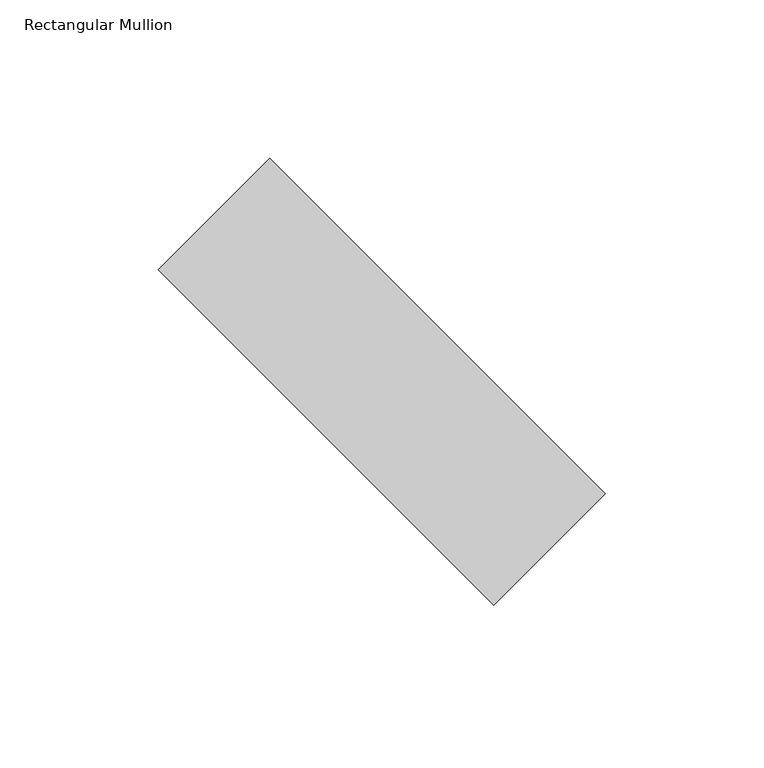
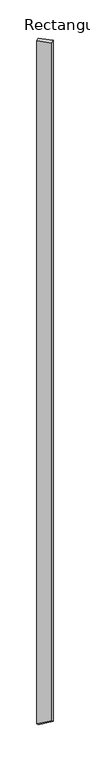
"""IFC4 building model written with IfcOpenShell, lengths in millimetres: member geometry, Rectangular Mullion : tilted mullions."""

from ifc_helpers import new_model, si_unit, origin, place, context, project, spatial, faceted_brep, source, transform, mapped, element, save


def rectangular_mullion_086599bb(model_context):
    return source(origin(), model_context, "Body", "Brep", [
        faceted_brep([(-35.3553391, 70.7106781, 0.0), (-70.7106781, 35.3553391, 0.0), (35.3553391, -70.7106781, 0.0), (70.7106781, -35.3553391, 0.0), (-35.3553391, 70.7106781, -8054.9932319), (-70.7106781, 35.3553391, -8010.0057806), (35.3553391, -70.7106781, -7944.5446238), (70.7106781, -35.3553391, -7989.532075)], [[[0, 1, 2, 3]], [[1, 0, 4, 5]], [[2, 1, 5, 6]], [[3, 2, 6, 7]], [[0, 3, 7, 4]], [[4, 7, 6, 5]]]),
    ])


if __name__ == "__main__":
    model = new_model("IFC4")
    model_context = context("Model", 3, world=origin())
    ifc_project = project(units=[si_unit("LENGTHUNIT", "METRE", prefix="MILLI")], contexts=[model_context])
    site = spatial("IfcSite", under=ifc_project)
    building = spatial("IfcBuilding", under=site)
    placement = place(None, origin())
    rectangular_mullion_shape = rectangular_mullion_086599bb(model_context)
    element("IfcMember", 1, ObjectType="Rectangular Mullion : tilted mullions", at=placement, inside=building, context=model_context, shape_type="MappedRepresentation", body=[
        mapped(rectangular_mullion_shape, transform((0.0, 0.0, 0.0), x_axis=(1.0, 0.0, 0.0), y_axis=(0.0, 1.0, 0.0), z_axis=(0.0, 0.0, 1.0))),
    ])
    save(model, "model.ifc")

# Revit data of these elements
# Type "Rectangular Mullion : tilted mullions"
#   built-in parameter 1007304 = 0.492126 (stored number, unit not read)
#   built-in parameter 1007301 = 0.082021 (stored number, unit not read)
#   built-in parameter 1007300 = 0.082021 (stored number, unit not read)
# Element 1 (IfcMember, "Rectangular Mullion : tilted mullions")
#   Materials on its faces: "Aluminum"
# Materials
#   "Aluminum": class "Metal", colour RGB 244 244 244, transparency 0, Description = "Aluminum 6061", Cost = 0
